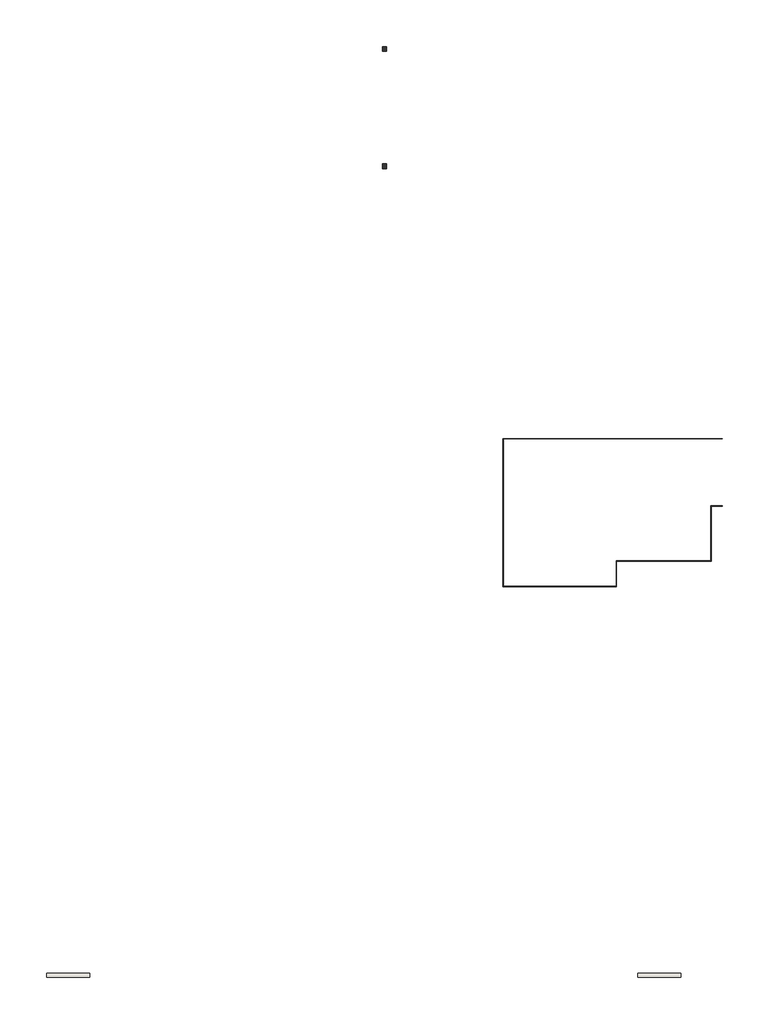
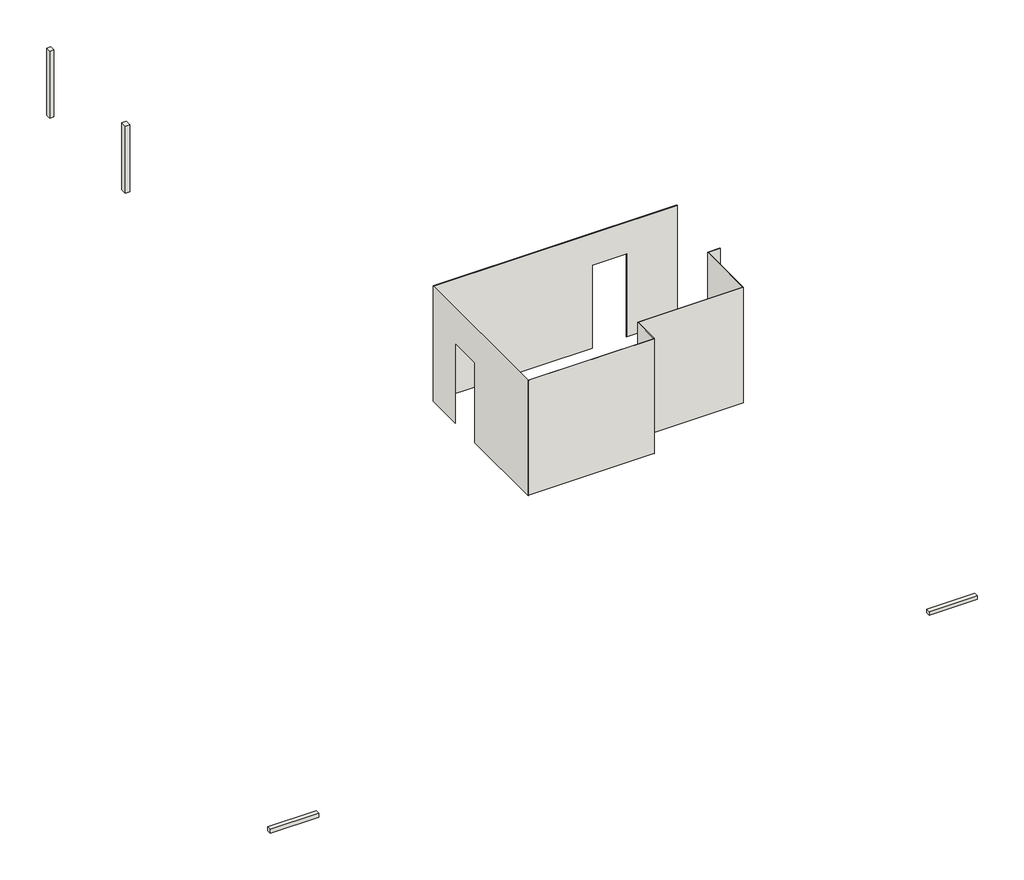
# One storey: 11 walls.
"""IFC4 building model written with IfcOpenShell, lengths in millimetres."""

import ifcopenshell
import ifcopenshell.guid

model = None  # the IFC model being written
_history = None  # IfcOwnerHistory: only IFC2X3 demands one
_inside = {}  # id of a spatial element -> (the spatial element, [elements in it])
_under = {}  # id of a project, library or spatial element -> (it, [spatial elements below it])
_declared = {}  # id of a project -> (the project, [libraries it declares])
_typed = {}  # id of a type object -> (the type object, [elements of that type])
_made_of = {}  # id of a material, layer set ... -> (it, [elements and type objects made of it])


def new_model(schema):
    """Start an empty IFC model of exactly this schema.

    Asked for "IFC4X3", IfcOpenShell would pick the latest addendum, in which some entities
    have other attributes; the version numbers below select the first issue.
    IFC2X3 requires an IfcOwnerHistory on every rooted entity: one is made here for all.
    """
    global model, _history
    if schema == "IFC4X3":
        model = ifcopenshell.file(schema_version=(4, 3, 0, 0))
    else:
        model = ifcopenshell.file(schema=schema)
    _inside.clear()
    _under.clear()
    _declared.clear()
    _typed.clear()
    _made_of.clear()
    _history = None
    if model.schema == "IFC2X3":
        org = make("IfcOrganization", Name="unknown")
        user = make(
            "IfcPersonAndOrganization",
            ThePerson=make("IfcPerson", FamilyName="unknown"),
            TheOrganization=org,
        )
        app = make(
            "IfcApplication",
            ApplicationDeveloper=org,
            Version="unknown",
            ApplicationFullName="unknown",
            ApplicationIdentifier="unknown",
        )
        _history = make(
            "IfcOwnerHistory",
            OwningUser=user,
            OwningApplication=app,
            ChangeAction="ADDED",
            CreationDate=0,
        )
    return model


def make(cls, **values):
    """One entity of the class cls with the attributes given. An attribute that is None is left unset."""
    return model.create_entity(
        cls, **{name: value for name, value in values.items() if value is not None}
    )


def rooted(cls, **values):
    """An entity with a GlobalId (a new one), such as an element, a storey or a relation."""
    return make(cls, GlobalId=ifcopenshell.guid.new(), OwnerHistory=_history, **values)


def si_unit(unit_type, name, prefix=None):
    """IfcSIUnit, for example si_unit("LENGTHUNIT", "METRE", prefix="MILLI")."""
    return make("IfcSIUnit", UnitType=unit_type, Prefix=prefix, Name=name)


def assignment(units):
    """IfcUnitAssignment: the units of a project."""
    return None if units is None else make("IfcUnitAssignment", Units=units)


def point(xyz):
    """IfcCartesianPoint."""
    return None if xyz is None else make("IfcCartesianPoint", Coordinates=xyz)


def direction(xyz):
    """IfcDirection."""
    return None if xyz is None else make("IfcDirection", DirectionRatios=xyz)


def frame(location, z_axis=None, x_axis=None):
    """IfcAxis2Placement3D, a coordinate frame: its origin and axes. An axis left out is left unset."""
    return make(
        "IfcAxis2Placement3D",
        Location=point(location),
        Axis=direction(z_axis),
        RefDirection=direction(x_axis),
    )


def origin():
    """The frame at (0, 0, 0) with its axes left unset."""
    return frame((0.0, 0.0, 0.0))


def place(relative_to, where):
    """IfcLocalPlacement: puts the frame where relative to a parent placement (None: the world)."""
    return make(
        "IfcLocalPlacement", PlacementRelTo=relative_to, RelativePlacement=where
    )


def context(
    kind, dimensions, precision=None, world=None, true_north=None, identifier=None
):
    """IfcGeometricRepresentationContext, for example the 3D "Model" context."""
    return make(
        "IfcGeometricRepresentationContext",
        ContextIdentifier=identifier,
        ContextType=kind,
        CoordinateSpaceDimension=dimensions,
        Precision=precision,
        WorldCoordinateSystem=world,
        TrueNorth=true_north,
    )


def project(units=None, contexts=None):
    """IfcProject with its units and contexts."""
    return rooted(
        "IfcProject",
        Name="project",
        RepresentationContexts=contexts,
        UnitsInContext=assignment(units),
    )


def spatial(cls, under=None, at=None, **own):
    """A site, building, storey or space (cls), placed at a placement, below another one or the project."""
    s = rooted(cls, ObjectPlacement=at, **own)
    if under is not None:
        _under.setdefault(under.id(), (under, []))[1].append(s)
    return s


def polyline(points):
    """IfcPolyline through the points."""
    return make("IfcPolyline", Points=[point(p) for p in points])


def outline(outer, holes=None, kind="AREA"):
    """IfcArbitraryClosedProfileDef: a profile drawn as a closed curve; with holes, ...WithVoids."""
    if holes is None:
        return make("IfcArbitraryClosedProfileDef", ProfileType=kind, OuterCurve=outer)
    return make(
        "IfcArbitraryProfileDefWithVoids",
        ProfileType=kind,
        OuterCurve=outer,
        InnerCurves=holes,
    )


def extrude(swept, where, along, depth):
    """IfcExtrudedAreaSolid: the profile swept, set in the frame where, extruded along a direction by depth."""
    return make(
        "IfcExtrudedAreaSolid",
        SweptArea=swept,
        Position=where,
        ExtrudedDirection=direction(along),
        Depth=depth,
    )


def faces_of(points, faces, orient=None, outer=None):
    """IfcFace entities. A face is a list of loops; a loop is a list of indices into points, from 0.

    orient and outer hold one flag for each loop. By default every Orientation is true, the
    first loop of a face is its IfcFaceOuterBound and the others are IfcFaceBound.
    """
    made = []
    for i, loops in enumerate(faces):
        bounds = []
        for j, loop in enumerate(loops):
            is_outer = j == 0 if outer is None else outer[i][j]
            bounds.append(
                make(
                    "IfcFaceOuterBound" if is_outer else "IfcFaceBound",
                    Bound=make("IfcPolyLoop", Polygon=[points[k] for k in loop]),
                    Orientation=True if orient is None else orient[i][j],
                )
            )
        made.append(make("IfcFace", Bounds=bounds))
    return made


def faceted_brep(points, faces, orient=None, outer=None, voids=None):
    """IfcFacetedBrep: a solid bounded by flat faces; with voids (closed shells), ...WithVoids."""
    shared = [point(p) for p in points]
    hull = make("IfcClosedShell", CfsFaces=faces_of(shared, faces, orient, outer))
    if voids is None:
        return make("IfcFacetedBrep", Outer=hull)
    return make(
        "IfcFacetedBrepWithVoids",
        Outer=hull,
        Voids=[
            make(cls, CfsFaces=faces_of(shared, fs, o, b)) for cls, fs, o, b in voids
        ],
    )


def shape(context_of_items, identifier, shape_type, items):
    """IfcShapeRepresentation: the items that make up one representation, for example the "Body"."""
    return make(
        "IfcShapeRepresentation",
        ContextOfItems=context_of_items,
        RepresentationIdentifier=identifier,
        RepresentationType=shape_type,
        Items=items,
    )


def made_of(thing, what):
    """Note that an element or type object is made of a material, layer set ...; save() writes the relation."""
    if what is not None:
        _made_of.setdefault(what.id(), (what, []))[1].append(thing)
    return thing


def element(
    cls,
    number,
    at=None,
    inside=None,
    cuts=None,
    type_object=None,
    material=None,
    context=None,
    identifier="Body",
    shape_type=None,
    held_by="IfcProductDefinitionShape",
    body=None,
    shapes=None,
    **own,
):
    """One element of the class cls, such as IfcWall. Its Tag is "e" and its number.

    at: its placement. inside: the storey or other place that contains it. cuts: it is an
    opening in that element (IfcRelVoidsElement). A single representation is given by context,
    identifier, shape_type and body (its items); several are given by shapes. held_by: the class
    of the entity that holds the representations. save() writes the other relations.
    """
    e = rooted(cls, Tag="e%d" % number, ObjectPlacement=at, **own)
    if body is not None:
        shapes = [shape(context, identifier, shape_type, body)]
    if shapes is not None:
        e.Representation = make(held_by, Representations=shapes)
    if inside is not None:
        _inside.setdefault(inside.id(), (inside, []))[1].append(e)
    if cuts is not None:
        rooted(
            "IfcRelVoidsElement", RelatingBuildingElement=cuts, RelatedOpeningElement=e
        )
    if type_object is not None:
        _typed.setdefault(type_object.id(), (type_object, []))[1].append(e)
    return made_of(e, material)


def aggregate(whole, parts):
    """IfcRelAggregates: a whole, such as a stair, and the parts it consists of."""
    return rooted("IfcRelAggregates", RelatingObject=whole, RelatedObjects=parts)


def save(model, path):
    """Write the relations noted so far, then the file.

    IfcRelAggregates (storeys below a building ...), IfcRelContainedInSpatialStructure (elements
    in a storey), IfcRelDefinesByType, IfcRelAssociatesMaterial and IfcRelDeclares: one each for
    every whole, place, type object, material and project.
    """
    for whole, parts in _under.values():
        aggregate(whole, parts)
    for where, things in _inside.values():
        rooted(
            "IfcRelContainedInSpatialStructure",
            RelatedElements=things,
            RelatingStructure=where,
        )
    for kind, things in _typed.values():
        rooted("IfcRelDefinesByType", RelatedObjects=things, RelatingType=kind)
    for what, things in _made_of.values():
        rooted("IfcRelAssociatesMaterial", RelatedObjects=things, RelatingMaterial=what)
    for by, libraries in _declared.values():
        rooted("IfcRelDeclares", RelatingContext=by, RelatedDefinitions=libraries)
    model.write(path)


model = new_model("IFC4")

# Units and contexts
model_context = context("Model", 3, world=origin())
ifc_project = project(units=[si_unit("LENGTHUNIT", "METRE", prefix="MILLI")], contexts=[model_context])

# Site, building, storey
site = spatial("IfcSite", under=ifc_project)
building = spatial("IfcBuilding", under=site)
storey = spatial("IfcBuildingStorey", under=building, Name="OK Türe 2.5m", Elevation=940.0)

# Walls
placement = place(None, origin())
element("IfcWall", 1, ObjectType="Alurahmen", at=placement, inside=storey, context=model_context, shape_type="SweptSolid", body=[
    extrude(outline(polyline([(72.7957948, 11869.149422), (72.7957948, 12024.149422), (202.7957948, 12024.149422), (202.7957948, 11869.149422), (72.7957948, 11869.149422)])), frame((0.0, 0.0, 940.0), z_axis=(0.0, 0.0, 1.0), x_axis=(1.0, 0.0, 0.0)), (0.0, 0.0, 1.0), 2097.6041168),
])
element("IfcWall", 2, ObjectType="Alurahmen", at=placement, inside=storey, context=model_context, shape_type="SweptSolid", body=[
    extrude(outline(polyline([(76.6105109, 8006.1476201), (76.6105109, 8176.1476201), (206.6105109, 8176.1476201), (206.6105109, 8006.1476201), (76.6105109, 8006.1476201)])), frame((0.0, 0.0, 940.0), z_axis=(0.0, 0.0, 1.0), x_axis=(1.0, 0.0, 0.0)), (0.0, 0.0, 1.0), 2097.6041168),
])
element("IfcWall", 3, ObjectType="Alurahmen 2", at=placement, inside=storey, context=model_context, shape_type="SweptSolid", body=[
    extrude(outline(polyline([(-9542.7075122, -18543.8567634), (-10969.1717517, -18543.8567634), (-10969.1717517, -18413.8567634), (-9542.7075122, -18413.8567634), (-9542.7075122, -18543.8567634)])), frame((0.0, 0.0, 940.0), z_axis=(0.0, 0.0, 1.0), x_axis=(1.0, 0.0, 0.0)), (0.0, 0.0, 1.0), 117.6041168),
])
element("IfcWall", 4, ObjectType="Alurahmen 2", at=placement, inside=storey, context=model_context, shape_type="SweptSolid", body=[
    extrude(outline(polyline([(9889.3842943, -18557.3276964), (8466.348791, -18557.3276964), (8466.348791, -18427.3276964), (9889.3842943, -18427.3276964), (9889.3842943, -18557.3276964)])), frame((0.0, 0.0, 940.0), z_axis=(0.0, 0.0, 1.0), x_axis=(1.0, 0.0, 0.0)), (0.0, 0.0, 1.0), 117.6041168),
])
element("IfcWall", 5, ObjectType="Fliesenspiegel Küche", at=placement, inside=storey, context=model_context, shape_type="Brep", body=[
    faceted_brep([(11241.7209992, -865.5726836, -1545.0), (11241.7209992, -865.5726836, 2037.6041168), (11238.3882373, -865.5726836, 2037.6041168), (11208.3882373, -865.5726836, 2037.6041168), (4041.7120809, -865.5726836, 2037.6041168), (4041.7120809, -865.5726836, -1545.0), (8733.2461289, -865.5726836, -1545.0), (8733.2461289, -865.5726836, 1045.9013429), (9748.2020231, -865.5726836, 1045.9013429), (9748.2020231, -865.5726836, -1545.0), (11208.3882373, -865.5726836, -1545.0), (11238.3882373, -865.5726836, -1545.0), (11241.7209992, -855.5726836, 2037.6041168), (11241.7209992, -855.5726836, -1545.0), (11238.3882373, -855.5726836, -1545.0), (11208.3882373, -855.5726836, -1545.0), (9748.2020231, -855.5726836, -1545.0), (9748.2020231, -855.5726836, 1045.9013429), (8733.2461289, -855.5726836, 1045.9013429), (8733.2461289, -855.5726836, -1545.0), (4041.7120721, -855.5726836, -1545.0), (4041.7120721, -855.5726836, 2037.6041168), (11208.3882373, -855.5726836, 2037.6041168), (11238.3882373, -855.5726836, 2037.6041168)], [[[0, 1, 2, 3, 4, 5, 6, 7, 8, 9, 10, 11]], [[12, 13, 14, 15, 16, 17, 18, 19, 20, 21, 22, 23]], [[13, 0, 11, 10, 9, 16, 15, 14]], [[5, 20, 19, 6]], [[1, 0, 13, 12]], [[4, 3, 2, 1, 12, 23, 22, 21]], [[5, 4, 21, 20]], [[7, 18, 17, 8]], [[18, 7, 6, 19]], [[8, 17, 16, 9]]]),
])
element("IfcWall", 6, ObjectType="Fliesenspiegel Küche", at=placement, inside=storey, context=model_context, shape_type="Brep", body=[
    faceted_brep([(4041.7163403, -5722.4101107, -1545.0), (7768.3882373, -5722.4101107, -1545.0), (7768.3882373, -5722.4101107, 2037.6041168), (4041.7163403, -5722.4101107, 2037.6041168), (4041.7163316, -5712.4101107, -1545.0), (4041.7163316, -5712.4101107, 2037.6041168), (7758.3882373, -5712.4101107, 2037.6041168), (7768.3882373, -5712.4101107, 2037.6041168), (7768.3882373, -5712.4101107, -1545.0), (7758.3882373, -5712.4101107, -1545.0), (7768.3882373, -5717.4101107, -1545.0)], [[[0, 1, 2, 3]], [[4, 5, 6, 7, 8, 9]], [[1, 0, 4, 9, 8, 10]], [[3, 2, 7, 6, 5]], [[0, 3, 5, 4]], [[2, 1, 10, 8, 7]]]),
])
element("IfcWall", 7, ObjectType="Fliesenspiegel Küche", at=placement, inside=storey, context=model_context, shape_type="SweptSolid", body=[
    extrude(outline(polyline([(-855.5726836, 2037.6041168), (-855.5726836, -1560.0), (-1982.7919385, -1560.0), (-1982.7919385, 937.4046304), (-2989.7013069, 937.4046304), (-2989.7013069, -1560.0), (-5712.4101107, -1560.0), (-5712.4101107, 2037.6041168), (-855.5726836, 2037.6041168)])), frame((4041.7173007, 0.0, 0.0), z_axis=(1.0, 0.0, 0.0), x_axis=(0.0, 1.0, 0.0)), (0.0, 0.0, 1.0), 10.0),
])
element("IfcWall", 8, ObjectType="Fliesenspiegel Küche", at=placement, inside=storey, context=model_context, shape_type="Brep", body=[
    faceted_brep([(7768.3882373, -5717.4101107, -1560.0), (7768.3882373, -5685.4101107, -1560.0), (7768.3882373, -4885.4101107, -1560.0), (7768.3882373, -4882.4101107, -1560.0), (7768.3882373, -4872.4101107, -1560.0), (7768.3882373, -4872.4101107, 2037.6041168), (7768.3882373, -4882.4101107, 2037.6041168), (7768.3882373, -5712.4101107, 2037.6041168), (7768.3882373, -5712.4101107, -1545.0), (7768.3882373, -5717.4101107, -1545.0), (7758.3882373, -5717.4101107, -1560.0), (7758.3882373, -5717.4101107, -1545.0), (7758.3882373, -5712.4101107, -1545.0), (7758.3882373, -5712.4101107, 2037.6041168), (7758.3882373, -4872.4101107, 2037.6041168), (7758.3882373, -4872.4101107, -1560.0)], [[[0, 1, 2, 3, 4, 5, 6, 7, 8, 9]], [[10, 11, 12, 13, 14, 15]], [[4, 3, 2, 1, 0, 10, 15]], [[7, 6, 5, 14, 13]], [[5, 4, 15, 14]], [[0, 9, 11, 10]], [[8, 12, 11, 9]], [[8, 7, 13, 12]]]),
])
element("IfcWall", 9, ObjectType="Fliesenspiegel Küche", at=placement, inside=storey, context=model_context, shape_type="Brep", body=[
    faceted_brep([(7768.3882373, -4882.4101107, -1560.0), (10878.3882373, -4882.4101107, -1560.0), (10878.3882373, -4882.4101107, 2037.6041168), (7768.3882373, -4882.4101107, 2037.6041168), (7768.3882373, -4872.4101107, -1560.0), (7768.3882373, -4872.4101107, 2037.6041168), (10868.3882373, -4872.4101107, 2037.6041168), (10878.3882373, -4872.4101107, 2037.6041168), (10878.3882373, -4872.4101107, -1545.0), (10878.3882373, -4872.4101107, -1560.0), (10878.3882373, -4877.4101107, -1560.0)], [[[0, 1, 2, 3]], [[4, 5, 6, 7, 8, 9]], [[1, 0, 4, 9, 10]], [[3, 2, 7, 6, 5]], [[0, 3, 5, 4]], [[2, 1, 10, 9, 8, 7]]]),
])
element("IfcWall", 10, ObjectType="Fliesenspiegel Küche", at=placement, inside=storey, context=model_context, shape_type="Brep", body=[
    faceted_brep([(10868.3882373, -3064.7705746, -1545.0), (10868.3882373, -4872.4101107, -1545.0), (10868.3882373, -4872.4101107, 2037.6041168), (10868.3882373, -3064.7705746, 2037.6041168), (10878.3882373, -3064.7705746, -1545.0), (10878.3882373, -3064.7705746, 2037.6041168), (10878.3882373, -3074.7705746, 2037.6041168), (10878.3882373, -4872.4101107, 2037.6041168), (10878.3882373, -4872.4101107, -1545.0), (10878.3882373, -3074.7705746, -1545.0)], [[[0, 1, 2, 3]], [[4, 5, 6, 7, 8, 9]], [[1, 0, 4, 9, 8]], [[3, 2, 7, 6, 5]], [[2, 1, 8, 7]], [[0, 3, 5, 4]]]),
])
element("IfcWall", 11, ObjectType="Fliesenspiegel Küche", at=placement, inside=storey, context=model_context, shape_type="Brep", body=[
    faceted_brep([(10878.3882373, -3074.7705746, -1545.0), (11238.3882373, -3074.7705746, -1545.0), (11238.3882373, -3074.7705746, 2037.6041168), (10878.3882373, -3074.7705746, 2037.6041168), (10878.3882373, -3064.7705746, -1545.0), (10878.3882373, -3064.7705746, 2037.6041168), (11208.3882373, -3064.7705746, 2037.6041168), (11238.3882373, -3064.7705746, 2037.6041168), (11238.3882373, -3064.7705746, -1545.0), (11208.3882373, -3064.7705746, -1545.0), (11238.3882373, -3069.7705746, -1545.0), (11238.3882373, -3069.7705746, 2037.6041168)], [[[0, 1, 2, 3]], [[4, 5, 6, 7, 8, 9]], [[1, 0, 4, 9, 8, 10]], [[3, 2, 11, 7, 6, 5]], [[2, 1, 10, 8, 7, 11]], [[0, 3, 5, 4]]]),
])

save(model, "model.ifc")

# Revit data of these elements
# Project information
#   Projektausgabedatum = "Projekt Datum"
#   Projektstatus = "Projektstatus"
#   Kundenname = "Bauherr"
#   Projektadresse = "Projektadresse"
#   Projektname = "Projektname"
#   Projektnummer = "Projektnummer"
#   Verfasser Firma 1 = "Firma 1"
#   Verfasser Firma 2 = "Firma 2"
#   Verfasser PLZ Ort = "PLZ Ort"
#   Verfasser Strasse = "Strasse"
#   Verfasser Telefon = "Telefon"
#   Verfasser Telefax = "Telefax"
#   Verfasser eMail = "E-Mail"
# Type "Alurahmen"
#   Type Comments = "Stahlbeton"
#   Description = "Stahlbeton 25.0 cm"
#   Layers, outside or top first: 0.130 m "Alumin." (function 1)
# Type "Alurahmen 2"
#   Type Comments = "Stahlbeton"
#   Description = "Stahlbeton 25.0 cm"
#   Layers, outside or top first: 0.130 m "Alumin." (function 1)
# Type "Fliesenspiegel Küche"
#   Type Comments = "Glasbaustein"
#   Description = "Glasbaustein 6.0 cm"
#   Layers, outside or top first: 0.010 m "Decke - Fliesen 25 x 25" (function 1)
# Elements 1, 2 (IfcWall, "Alurahmen")
#   Top Offset = 0.000 m
#   Base Offset = 0.000 m
#   wall height = 2.097604 m
#   Phase Created = Phase 1
#   Base Constraint = OK Türe 2.5m
#   Top Constraint = Ebene 1 OK Wand
#   Materials on its faces: "Alumin."
# Elements 3, 4 (IfcWall, "Alurahmen 2")
#   Top Offset = -1.980 m
#   Base Offset = 0.000 m
#   wall height = 0.117604 m
#   Phase Created = Phase 1
#   Base Constraint = OK Türe 2.5m
#   Top Constraint = Ebene 1 OK Wand
#   Materials on its faces: "Alumin."
# Elements 5, 6, 10 (IfcWall, "Fliesenspiegel Küche")
#   built-in parameter 1001111 = -2.485 m
#   Top Offset = 0.300 m
#   Base Offset = -2.485 m
#   wall height = 3.582604 m
#   Phase Created = Phase 1
#   Base Constraint = OK Türe 2.5m
#   Top Constraint = UK Unterzug 1.30
#   Materials on its faces: "Decke - Fliesen 25 x 25"
# Elements 7, 8, 9 (IfcWall, "Fliesenspiegel Küche")
#   built-in parameter 1001111 = -2.500 m
#   Top Offset = 0.300 m
#   Base Offset = -2.500 m
#   wall height = 3.597604 m
#   Phase Created = Phase 1
#   Base Constraint = OK Türe 2.5m
#   Top Constraint = UK Unterzug 1.30
#   Materials on its faces: "Decke - Fliesen 25 x 25"
# Element 11 (IfcWall, "Fliesenspiegel Küche")
#   built-in parameter 1001111 = -2.485 m
#   Top Offset = 0.300 m
#   Base Offset = -2.485 m
#   wall height = 3.582604 m
#   Phase Created = Phase 1
#   Base Constraint = OK Türe 2.5m
#   Top Constraint = UK Unterzug 1.30
#   Materials on its faces: "Decke - Fliesen 25 x 25", "Glas - Klar"
# Materials
#   "Alumin.": class "Metall", colour RGB 247 247 247, transparency 0, Description = "Aluminium 6061", Cost = 0
#   "Decke - Fliesen 25 x 25": class "Keramik", colour RGB 125 125 125, transparency 0, Cost = 0
#   "Glas - Klar": class "Glas", colour RGB 128 128 255, transparency 0.75, Cost = 0
